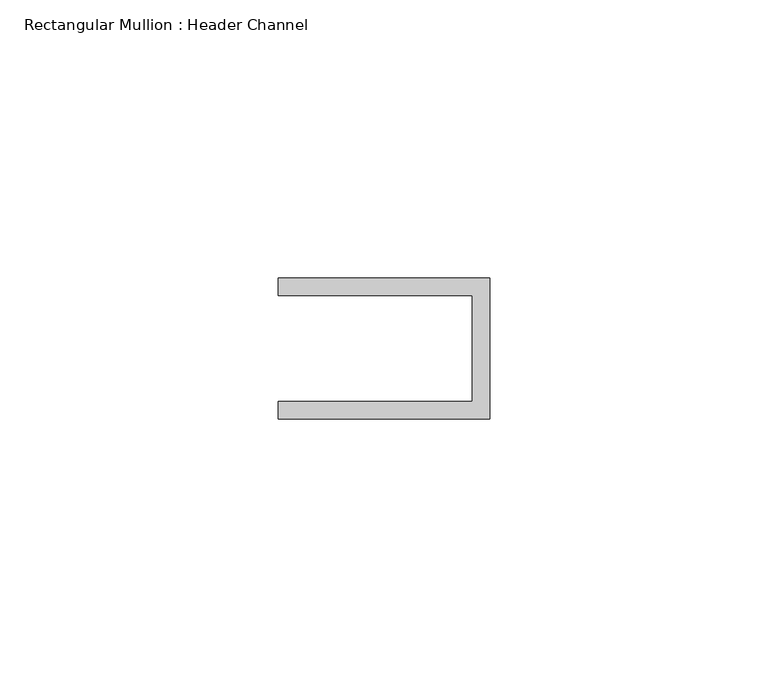
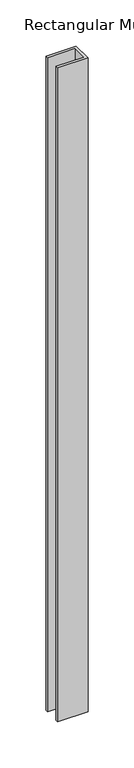
"""IFC4 building model written with IfcOpenShell, lengths in millimetres: member geometry, Rectangular Mullion : Header Channel."""

from ifc_helpers import new_model, si_unit, frame, origin, place, context, project, spatial, polyline, outline, extrude, source, transform, mapped, element, save


def rectangular_mullion_header_channel_94ec25d3(model_context):
    return source(origin(), model_context, "Body", "SweptSolid", [
        extrude(outline(polyline([(0.0, 12.7), (0.0, -12.7), (-38.1, -12.7), (-38.1, -9.525), (-3.175, -9.525), (-3.175, 9.525), (-38.1, 9.525), (-38.1, 12.7), (0.0, 12.7)])), frame((0.0, 0.0, -866.775), z_axis=(0.0, 0.0, 1.0), x_axis=(1.0, 0.0, 0.0)), (0.0, 0.0, 1.0), 866.775),
    ])


if __name__ == "__main__":
    model = new_model("IFC4")
    model_context = context("Model", 3, world=origin())
    ifc_project = project(units=[si_unit("LENGTHUNIT", "METRE", prefix="MILLI")], contexts=[model_context])
    site = spatial("IfcSite", under=ifc_project)
    building = spatial("IfcBuilding", under=site)
    placement = place(None, origin())
    rectangular_mullion_header_channel_shape = rectangular_mullion_header_channel_94ec25d3(model_context)
    element("IfcMember", 1, ObjectType="Rectangular Mullion : Header Channel", at=placement, inside=building, context=model_context, shape_type="MappedRepresentation", body=[
        mapped(rectangular_mullion_header_channel_shape, transform((0.0, 0.0, 0.0), x_axis=(1.0, 0.0, 0.0), y_axis=(0.0, 1.0, 0.0), z_axis=(0.0, 0.0, 1.0))),
    ])
    save(model, "model.ifc")

# Revit data of these elements
# Type "Rectangular Mullion : Header Channel"
#   built-in parameter 1007322 = 0.0833333 (stored number, unit not read)
#   built-in parameter 1007321 = -0.03125 (stored number, unit not read)
#   built-in parameter 1007320 = 0.0416667 (stored number, unit not read)
# Element 1 (IfcMember, "Rectangular Mullion : Header Channel")
#   Materials on its faces: "ALUM"
# Materials
#   "ALUM": class "Generic", colour RGB 157 157 157, transparency 0, Cost = 0
